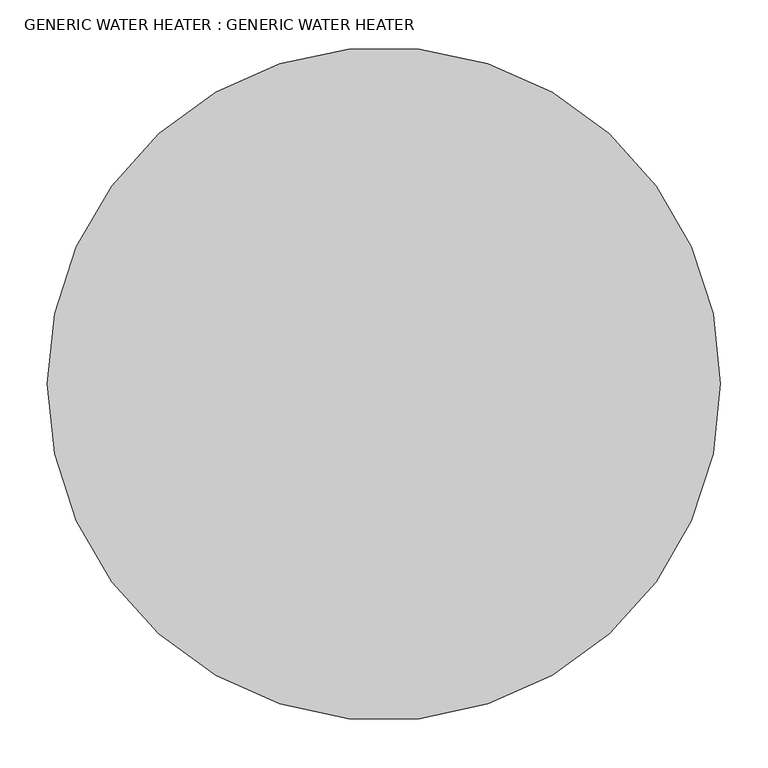
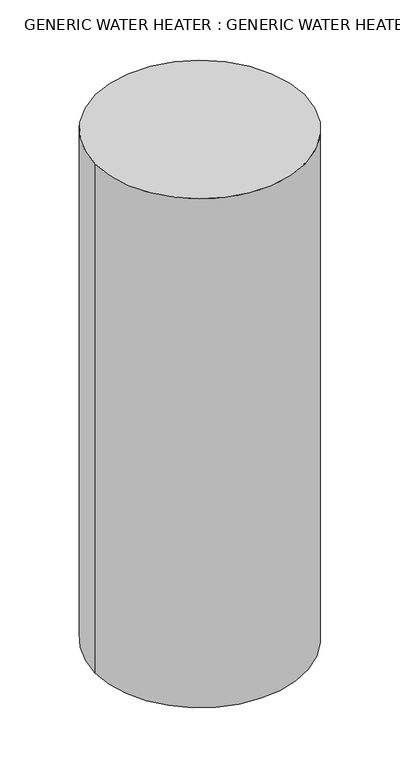
"""IFC4 building model written with IfcOpenShell, lengths in millimetres: proxy geometry, GENERIC WATER HEATER : GENERIC WATER HEATER."""

import ifcopenshell
import ifcopenshell.guid

model = None  # the IFC model being written
_history = None  # IfcOwnerHistory: only IFC2X3 demands one
_inside = {}  # id of a spatial element -> (the spatial element, [elements in it])
_under = {}  # id of a project, library or spatial element -> (it, [spatial elements below it])
_declared = {}  # id of a project -> (the project, [libraries it declares])
_typed = {}  # id of a type object -> (the type object, [elements of that type])
_made_of = {}  # id of a material, layer set ... -> (it, [elements and type objects made of it])


def new_model(schema):
    """Start an empty IFC model of exactly this schema.

    Asked for "IFC4X3", IfcOpenShell would pick the latest addendum, in which some entities
    have other attributes; the version numbers below select the first issue.
    IFC2X3 requires an IfcOwnerHistory on every rooted entity: one is made here for all.
    """
    global model, _history
    if schema == "IFC4X3":
        model = ifcopenshell.file(schema_version=(4, 3, 0, 0))
    else:
        model = ifcopenshell.file(schema=schema)
    _inside.clear()
    _under.clear()
    _declared.clear()
    _typed.clear()
    _made_of.clear()
    _history = None
    if model.schema == "IFC2X3":
        org = make("IfcOrganization", Name="unknown")
        user = make(
            "IfcPersonAndOrganization",
            ThePerson=make("IfcPerson", FamilyName="unknown"),
            TheOrganization=org,
        )
        app = make(
            "IfcApplication",
            ApplicationDeveloper=org,
            Version="unknown",
            ApplicationFullName="unknown",
            ApplicationIdentifier="unknown",
        )
        _history = make(
            "IfcOwnerHistory",
            OwningUser=user,
            OwningApplication=app,
            ChangeAction="ADDED",
            CreationDate=0,
        )
    return model


def make(cls, **values):
    """One entity of the class cls with the attributes given. An attribute that is None is left unset."""
    return model.create_entity(
        cls, **{name: value for name, value in values.items() if value is not None}
    )


def rooted(cls, **values):
    """An entity with a GlobalId (a new one), such as an element, a storey or a relation."""
    return make(cls, GlobalId=ifcopenshell.guid.new(), OwnerHistory=_history, **values)


def si_unit(unit_type, name, prefix=None):
    """IfcSIUnit, for example si_unit("LENGTHUNIT", "METRE", prefix="MILLI")."""
    return make("IfcSIUnit", UnitType=unit_type, Prefix=prefix, Name=name)


def assignment(units):
    """IfcUnitAssignment: the units of a project."""
    return None if units is None else make("IfcUnitAssignment", Units=units)


def point(xyz):
    """IfcCartesianPoint."""
    return None if xyz is None else make("IfcCartesianPoint", Coordinates=xyz)


def direction(xyz):
    """IfcDirection."""
    return None if xyz is None else make("IfcDirection", DirectionRatios=xyz)


def frame(location, z_axis=None, x_axis=None):
    """IfcAxis2Placement3D, a coordinate frame: its origin and axes. An axis left out is left unset."""
    return make(
        "IfcAxis2Placement3D",
        Location=point(location),
        Axis=direction(z_axis),
        RefDirection=direction(x_axis),
    )


def frame_2d(location, x_axis=None):
    """IfcAxis2Placement2D, a coordinate frame in the plane: its origin and x axis."""
    return make(
        "IfcAxis2Placement2D", Location=point(location), RefDirection=direction(x_axis)
    )


def origin():
    """The frame at (0, 0, 0) with its axes left unset."""
    return frame((0.0, 0.0, 0.0))


def origin_with_axes():
    """The frame at (0, 0, 0) with the z axis (0, 0, 1) and the x axis (1, 0, 0) written out."""
    return frame((0.0, 0.0, 0.0), z_axis=(0.0, 0.0, 1.0), x_axis=(1.0, 0.0, 0.0))


def origin_2d():
    """The frame at (0, 0) in the plane with its x axis left unset."""
    return frame_2d((0.0, 0.0))


def place(relative_to, where):
    """IfcLocalPlacement: puts the frame where relative to a parent placement (None: the world)."""
    return make(
        "IfcLocalPlacement", PlacementRelTo=relative_to, RelativePlacement=where
    )


def context(
    kind, dimensions, precision=None, world=None, true_north=None, identifier=None
):
    """IfcGeometricRepresentationContext, for example the 3D "Model" context."""
    return make(
        "IfcGeometricRepresentationContext",
        ContextIdentifier=identifier,
        ContextType=kind,
        CoordinateSpaceDimension=dimensions,
        Precision=precision,
        WorldCoordinateSystem=world,
        TrueNorth=true_north,
    )


def project(units=None, contexts=None):
    """IfcProject with its units and contexts."""
    return rooted(
        "IfcProject",
        Name="project",
        RepresentationContexts=contexts,
        UnitsInContext=assignment(units),
    )


def spatial(cls, under=None, at=None, **own):
    """A site, building, storey or space (cls), placed at a placement, below another one or the project."""
    s = rooted(cls, ObjectPlacement=at, **own)
    if under is not None:
        _under.setdefault(under.id(), (under, []))[1].append(s)
    return s


def circle_curve(where, radius):
    """IfcCircle in the frame where."""
    return make("IfcCircle", Position=where, Radius=radius)


def trimmed(basis, trim1, trim2, sense, master):
    """IfcTrimmedCurve: the piece of a basis curve between two trims."""
    return make(
        "IfcTrimmedCurve",
        BasisCurve=basis,
        Trim1=trim1,
        Trim2=trim2,
        SenseAgreement=sense,
        MasterRepresentation=master,
    )


def segment(curve, same_sense, transition):
    """IfcCompositeCurveSegment."""
    return make(
        "IfcCompositeCurveSegment",
        Transition=transition,
        SameSense=same_sense,
        ParentCurve=curve,
    )


def composite_curve(segments, self_intersect=None):
    """IfcCompositeCurve: segments joined end to end."""
    return make("IfcCompositeCurve", Segments=segments, SelfIntersect=self_intersect)


def outline(outer, holes=None, kind="AREA"):
    """IfcArbitraryClosedProfileDef: a profile drawn as a closed curve; with holes, ...WithVoids."""
    if holes is None:
        return make("IfcArbitraryClosedProfileDef", ProfileType=kind, OuterCurve=outer)
    return make(
        "IfcArbitraryProfileDefWithVoids",
        ProfileType=kind,
        OuterCurve=outer,
        InnerCurves=holes,
    )


def extrude(swept, where, along, depth):
    """IfcExtrudedAreaSolid: the profile swept, set in the frame where, extruded along a direction by depth."""
    return make(
        "IfcExtrudedAreaSolid",
        SweptArea=swept,
        Position=where,
        ExtrudedDirection=direction(along),
        Depth=depth,
    )


def shape(context_of_items, identifier, shape_type, items):
    """IfcShapeRepresentation: the items that make up one representation, for example the "Body"."""
    return make(
        "IfcShapeRepresentation",
        ContextOfItems=context_of_items,
        RepresentationIdentifier=identifier,
        RepresentationType=shape_type,
        Items=items,
    )


def source(mapping_origin, context_of_items, identifier, shape_type, items):
    """IfcRepresentationMap: a shape defined once, which mapped items show again and again."""
    return make(
        "IfcRepresentationMap",
        MappingOrigin=mapping_origin,
        MappedRepresentation=shape(context_of_items, identifier, shape_type, items),
    )


def transform(
    local_origin,
    x_axis=None,
    y_axis=None,
    z_axis=None,
    scale=None,
    scale2=None,
    scale3=None,
    uniform=True,
):
    """IfcCartesianTransformationOperator3D, or its non-uniform kind. x_axis, y_axis, z_axis: its Axis1, 2, 3."""
    if uniform:
        return make(
            "IfcCartesianTransformationOperator3D",
            Axis1=direction(x_axis),
            Axis2=direction(y_axis),
            LocalOrigin=point(local_origin),
            Scale=scale,
            Axis3=direction(z_axis),
        )
    return make(
        "IfcCartesianTransformationOperator3DnonUniform",
        Axis1=direction(x_axis),
        Axis2=direction(y_axis),
        LocalOrigin=point(local_origin),
        Scale=scale,
        Axis3=direction(z_axis),
        Scale2=scale2,
        Scale3=scale3,
    )


def mapped(mapping_source, mapping_target):
    """IfcMappedItem: shows the shape of a source again, moved by a transform."""
    return make(
        "IfcMappedItem", MappingSource=mapping_source, MappingTarget=mapping_target
    )


def made_of(thing, what):
    """Note that an element or type object is made of a material, layer set ...; save() writes the relation."""
    if what is not None:
        _made_of.setdefault(what.id(), (what, []))[1].append(thing)
    return thing


def element(
    cls,
    number,
    at=None,
    inside=None,
    cuts=None,
    type_object=None,
    material=None,
    context=None,
    identifier="Body",
    shape_type=None,
    held_by="IfcProductDefinitionShape",
    body=None,
    shapes=None,
    **own,
):
    """One element of the class cls, such as IfcWall. Its Tag is "e" and its number.

    at: its placement. inside: the storey or other place that contains it. cuts: it is an
    opening in that element (IfcRelVoidsElement). A single representation is given by context,
    identifier, shape_type and body (its items); several are given by shapes. held_by: the class
    of the entity that holds the representations. save() writes the other relations.
    """
    e = rooted(cls, Tag="e%d" % number, ObjectPlacement=at, **own)
    if body is not None:
        shapes = [shape(context, identifier, shape_type, body)]
    if shapes is not None:
        e.Representation = make(held_by, Representations=shapes)
    if inside is not None:
        _inside.setdefault(inside.id(), (inside, []))[1].append(e)
    if cuts is not None:
        rooted(
            "IfcRelVoidsElement", RelatingBuildingElement=cuts, RelatedOpeningElement=e
        )
    if type_object is not None:
        _typed.setdefault(type_object.id(), (type_object, []))[1].append(e)
    return made_of(e, material)


def aggregate(whole, parts):
    """IfcRelAggregates: a whole, such as a stair, and the parts it consists of."""
    return rooted("IfcRelAggregates", RelatingObject=whole, RelatedObjects=parts)


def save(model, path):
    """Write the relations noted so far, then the file.

    IfcRelAggregates (storeys below a building ...), IfcRelContainedInSpatialStructure (elements
    in a storey), IfcRelDefinesByType, IfcRelAssociatesMaterial and IfcRelDeclares: one each for
    every whole, place, type object, material and project.
    """
    for whole, parts in _under.values():
        aggregate(whole, parts)
    for where, things in _inside.values():
        rooted(
            "IfcRelContainedInSpatialStructure",
            RelatedElements=things,
            RelatingStructure=where,
        )
    for kind, things in _typed.values():
        rooted("IfcRelDefinesByType", RelatedObjects=things, RelatingType=kind)
    for what, things in _made_of.values():
        rooted("IfcRelAssociatesMaterial", RelatedObjects=things, RelatingMaterial=what)
    for by, libraries in _declared.values():
        rooted("IfcRelDeclares", RelatingContext=by, RelatedDefinitions=libraries)
    model.write(path)


def generic_water_heater_generic_water_heater_aa4aec31(model_context):
    return source(origin(), model_context, "Body", "SweptSolid", [
        extrude(outline(composite_curve([segment(trimmed(circle_curve(origin_2d(), 355.6), [point((-355.6, 0.0))], [point((355.6, 0.0))], False, "CARTESIAN"), True, "CONTINUOUS"), segment(trimmed(circle_curve(origin_2d(), 355.6), [point((355.6, 0.0))], [point((-355.6, 0.0))], False, "CARTESIAN"), True, "CONTINUOUS")], self_intersect=False)), origin_with_axes(), (0.0, 0.0, 1.0), 1828.8),
    ])


if __name__ == "__main__":
    model = new_model("IFC4")
    model_context = context("Model", 3, world=origin())
    ifc_project = project(units=[si_unit("LENGTHUNIT", "METRE", prefix="MILLI")], contexts=[model_context])
    site = spatial("IfcSite", under=ifc_project)
    building = spatial("IfcBuilding", under=site)
    placement = place(None, origin())
    generic_water_heater_generic_water_heater_shape = generic_water_heater_generic_water_heater_aa4aec31(model_context)
    element("IfcBuildingElementProxy", 1, Name="GENERIC WATER HEATER : GENERIC WATER HEATER", ObjectType="GENERIC WATER HEATER : GENERIC WATER HEATER", at=placement, inside=building, context=model_context, shape_type="MappedRepresentation", body=[
        mapped(generic_water_heater_generic_water_heater_shape, transform((0.0, 0.0, 0.0), x_axis=(1.0, 0.0, 0.0), y_axis=(0.0, 1.0, 0.0), z_axis=(0.0, 0.0, 1.0))),
    ])
    save(model, "model.ifc")
